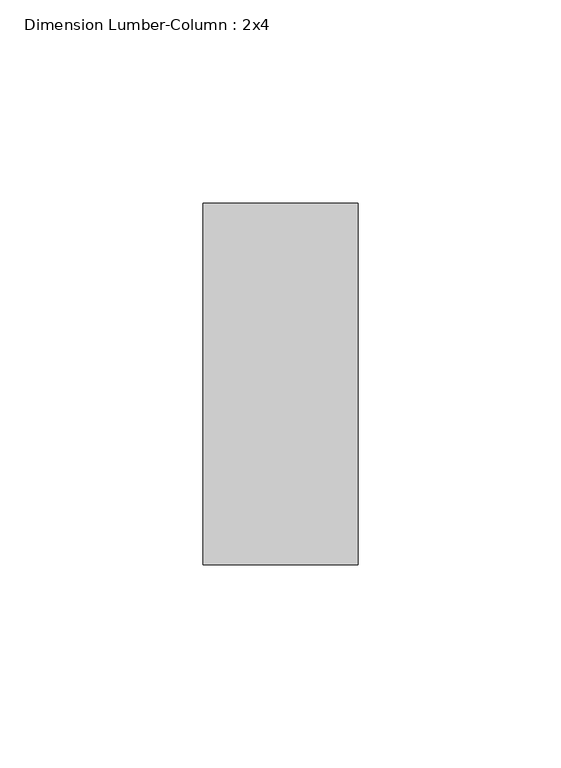
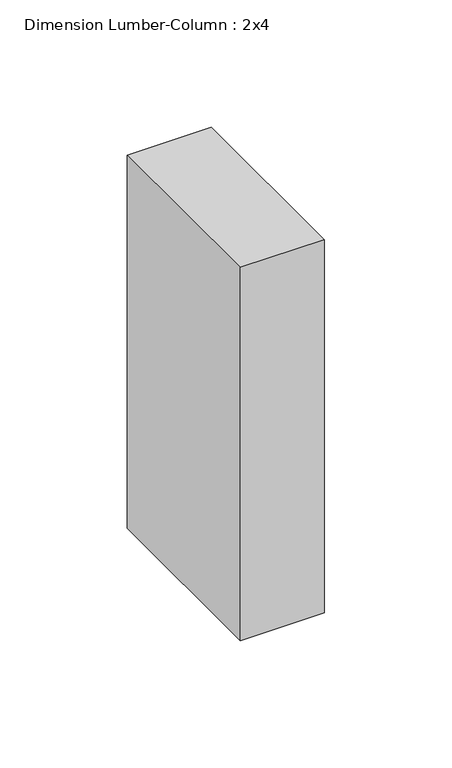
"""IFC4 building model written with IfcOpenShell, lengths in millimetres: column geometry, Dimension Lumber-Column : 2x4."""

from ifc_helpers import new_model, si_unit, frame, origin, place, context, project, spatial, polyline, outline, extrude, source, transform, mapped, element, save


def dimension_lumber_column_2x4_1a929157(model_context):
    return source(origin(), model_context, "Body", "SweptSolid", [
        extrude(outline(polyline([(19.05, 44.45), (19.05, -44.45), (-19.05, -44.45), (-19.05, 44.45), (19.05, 44.45)])), frame((0.0, 0.0, 2208.609375), z_axis=(0.0, 0.0, 1.0), x_axis=(1.0, 0.0, 0.0)), (0.0, 0.0, 1.0), 178.990625),
    ])


if __name__ == "__main__":
    model = new_model("IFC4")
    model_context = context("Model", 3, world=origin())
    ifc_project = project(units=[si_unit("LENGTHUNIT", "METRE", prefix="MILLI")], contexts=[model_context])
    site = spatial("IfcSite", under=ifc_project)
    building = spatial("IfcBuilding", under=site)
    placement = place(None, origin())
    dimension_lumber_column_2x4_shape = dimension_lumber_column_2x4_1a929157(model_context)
    element("IfcColumn", 1, ObjectType="Dimension Lumber-Column : 2x4", at=placement, inside=building, context=model_context, shape_type="MappedRepresentation", body=[
        mapped(dimension_lumber_column_2x4_shape, transform((0.0, 0.0, 0.0), x_axis=(1.0, 0.0, 0.0), y_axis=(0.0, 1.0, 0.0), z_axis=(0.0, 0.0, 1.0))),
    ])
    save(model, "model.ifc")

# Revit data of these elements
# Type "Dimension Lumber-Column : 2x4"
#   Int Type = "Interior"
#   Assembly Code = "B10"
#   Cost = 8.05
#   A = 0.0364583 SF
#   b = 0' - 1 1/2"
#   d = 0' - 3 1/2"
#   Structural Material [instance default] = Softwood, Lumber
# Element 1 (IfcColumn, "Dimension Lumber-Column : 2x4")
#   Structural Material = Douglas Fir #2
#   Materials on its faces: "Douglas Fir #2"
# Materials
#   "Softwood, Lumber": class "Wood", colour RGB 223 192 134, transparency 0, Description = "Pinus Echinata", Cost = 0
#   "Douglas Fir #2": class "Wood", colour RGB 223 192 134, transparency 0, Description = "Pinus Echinata", Cost = 0
